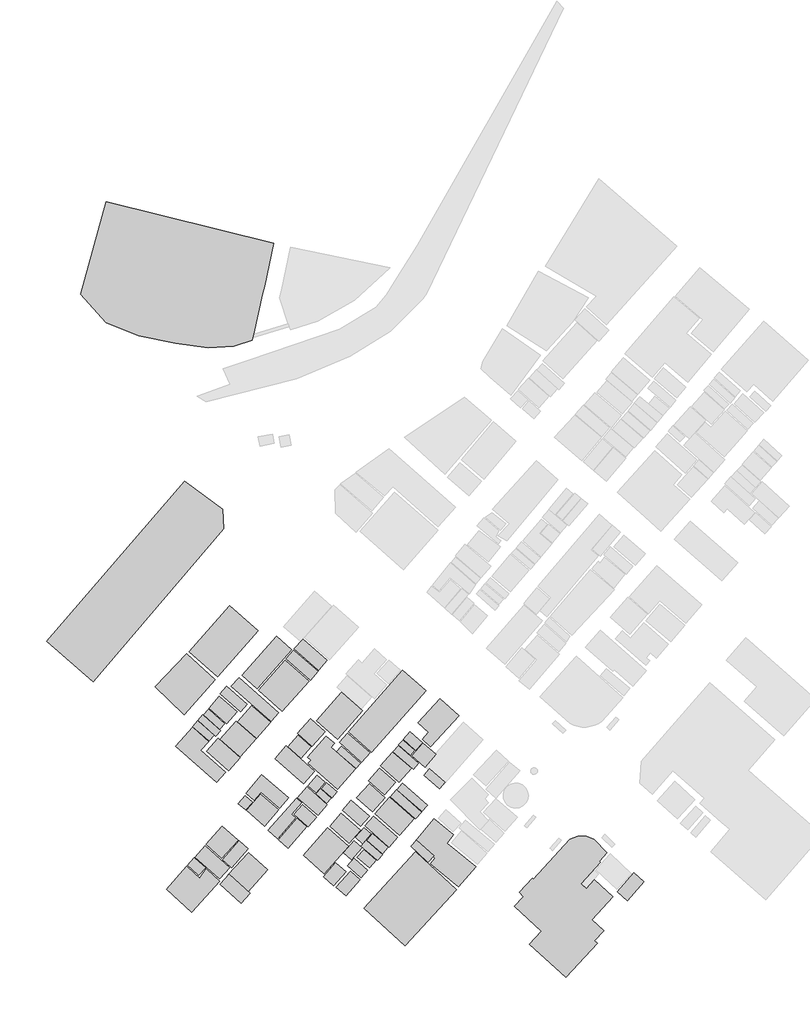
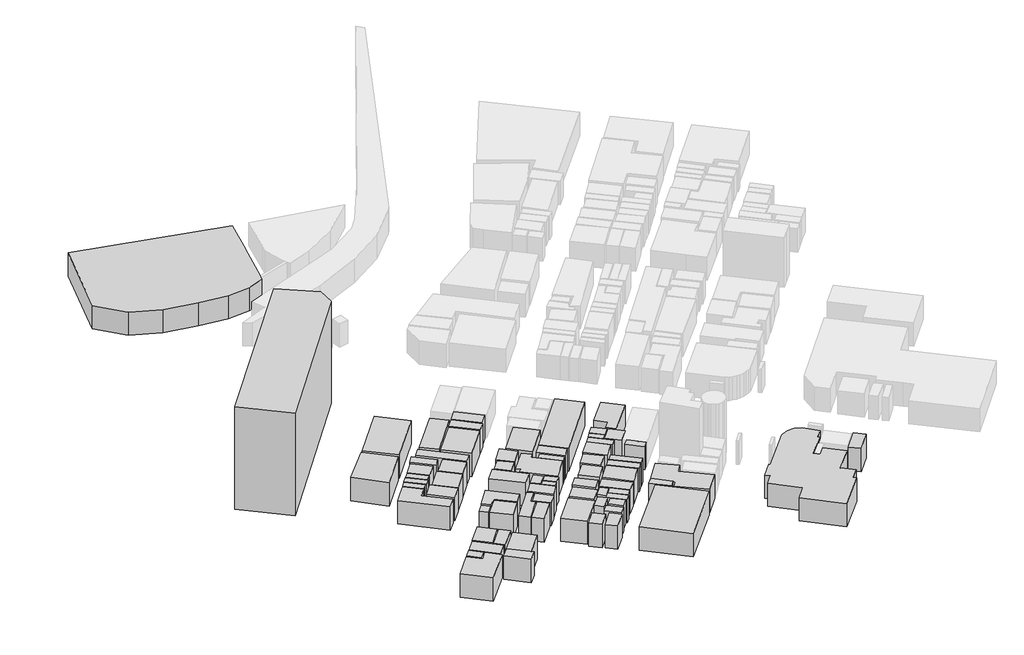
# Not in any storey, part 1 of 3: 72 proxies.
"""IFC4 building model written with IfcOpenShell, lengths in millimetres."""

from ifc_helpers import new_model, si_unit, origin, origin_with_axes, place, context, project, spatial, polyline, outline, extrude, element, save

model = new_model("IFC4")

# Units and contexts
model_context = context("Model", 3, world=origin())
ifc_project = project(units=[si_unit("LENGTHUNIT", "METRE", prefix="MILLI")], contexts=[model_context])

# Site, building
site = spatial("IfcSite", under=ifc_project)
building = spatial("IfcBuilding", under=site)

# Proxies
placement = place(None, origin())
element("IfcBuildingElementProxy", 1, Name="Mass", at=placement, inside=building, context=model_context, shape_type="SweptSolid", body=[
    extrude(outline(polyline([(-81027.0217269, 125127.6509537), (-8762.1194073, 208768.4747751), (11065.563168, 193957.3105467), (11679.8148372, 183871.9306999), (-56475.0211631, 103911.6589493), (-81027.0217269, 125127.6509537)])), origin_with_axes(), (0.0, 0.0, 1.0), 66000.0),
])
element("IfcBuildingElementProxy", 2, Name="Mass", at=placement, inside=building, context=model_context, shape_type="SweptSolid", body=[
    extrude(outline(polyline([(60169.5642931, 83373.9559982), (73321.7765149, 98307.4346465), (84306.0416675, 88633.4760284), (71144.7963334, 73699.9973801), (60169.5642931, 83373.9559982)])), origin_with_axes(), (0.0, 0.0, 1.0), 15000.0),
])
element("IfcBuildingElementProxy", 3, Name="Mass", at=placement, inside=building, context=model_context, shape_type="SweptSolid", body=[
    extrude(outline(polyline([(2438.9404523, 18836.4205741), (10893.9340249, 28276.8698459), (19105.0335488, 20926.8851949), (10650.0399787, 11475.3164303), (2438.9404523, 18836.4205741)])), origin_with_axes(), (0.0, 0.0, 1.0), 15000.0),
])
element("IfcBuildingElementProxy", 4, Name="Mass", at=placement, inside=building, context=model_context, shape_type="SweptSolid", body=[
    extrude(outline(polyline([(85191.2867223, 27565.2223158), (88867.7636278, 24318.3304577), (84405.4059075, 19258.9612947), (80728.929002, 22494.7336608), (85191.2867223, 27565.2223158)])), origin_with_axes(), (0.0, 0.0, 1.0), 15000.0),
])
element("IfcBuildingElementProxy", 5, Name="Mass", at=placement, inside=building, context=model_context, shape_type="SweptSolid", body=[
    extrude(outline(polyline([(76944.0547443, 77691.8952467), (105371.2606935, 109960.6629591), (117538.8636232, 99230.3525382), (89120.6907837, 66972.7043185), (76944.0547443, 77691.8952467)])), origin_with_axes(), (0.0, 0.0, 1.0), 15000.0),
])
element("IfcBuildingElementProxy", 6, Name="Mass", at=placement, inside=building, context=model_context, shape_type="SweptSolid", body=[
    extrude(outline(polyline([(105479.6580482, 73344.1736146), (111622.1747453, 67928.9806877), (109400.0289974, 65415.9753454), (103248.4791881, 70820.0487803), (105479.6580482, 73344.1736146)])), origin_with_axes(), (0.0, 0.0, 1.0), 15000.0),
])
element("IfcBuildingElementProxy", 7, Name="Mass", at=placement, inside=building, context=model_context, shape_type="SweptSolid", body=[
    extrude(outline(polyline([(65986.8889311, 27531.8638374), (76907.9222927, 17913.5026824), (64279.6306124, 3580.4766379), (53358.5972507, 13198.8377929), (65986.8889311, 27531.8638374)])), origin_with_axes(), (0.0, 0.0, 1.0), 15000.0),
])
element("IfcBuildingElementProxy", 8, Name="Mass", at=placement, inside=building, context=model_context, shape_type="SweptSolid", body=[
    extrude(outline(polyline([(81496.7435898, 12142.4859901), (85010.6244644, 16134.3838566), (91424.1345471, 10485.6815827), (87910.2536699, 6493.7837161), (81496.7435898, 12142.4859901)])), origin_with_axes(), (0.0, 0.0, 1.0), 15000.0),
])
element("IfcBuildingElementProxy", 9, Name="Mass", at=placement, inside=building, context=model_context, shape_type="SweptSolid", body=[
    extrude(outline(polyline([(-1878.8874617, 83362.8365054), (6657.4041263, 75834.9399721), (4082.96698, 72910.5134012), (-4453.3246055, 80427.2904425), (-1878.8874617, 83362.8365054)])), origin_with_axes(), (0.0, 0.0, 1.0), 15000.0),
])
element("IfcBuildingElementProxy", 10, Name="Mass", at=placement, inside=building, context=model_context, shape_type="SweptSolid", body=[
    extrude(outline(polyline([(3676.4769055, 89478.5574712), (12266.9671671, 81906.1829667), (9674.4637962, 78970.636903), (1083.9735346, 86543.0114075), (3676.4769055, 89478.5574712)])), origin_with_axes(), (0.0, 0.0, 1.0), 15000.0),
])
element("IfcBuildingElementProxy", 11, Name="Mass", at=placement, inside=building, context=model_context, shape_type="SweptSolid", body=[
    extrude(outline(polyline([(13179.3115586, 101509.8485342), (23883.550216, 92080.5187543), (20514.1991451, 88266.5327709), (9818.9936026, 97695.8625499), (13179.3115586, 101509.8485342)])), origin_with_axes(), (0.0, 0.0, 1.0), 15000.0),
])
element("IfcBuildingElementProxy", 12, Name="Mass", at=placement, inside=building, context=model_context, shape_type="SweptSolid", body=[
    extrude(outline(polyline([(62762.0676639, 48025.088818), (65499.1008385, 51127.4272713), (70982.2003026, 46290.4479627), (68245.167128, 43188.1095094), (62762.0676639, 48025.088818)])), origin_with_axes(), (0.0, 0.0, 1.0), 15000.0),
])
element("IfcBuildingElementProxy", 13, Name="Mass", at=placement, inside=building, context=model_context, shape_type="SweptSolid", body=[
    extrude(outline(polyline([(18174.6229327, 83262.7610719), (28625.9344316, 74066.9406383), (20342.570002, 64670.9693369), (9900.291618, 73877.9092632), (18174.6229327, 83262.7610719)])), origin_with_axes(), (0.0, 0.0, 1.0), 15000.0),
])
element("IfcBuildingElementProxy", 14, Name="Mass", at=placement, inside=building, context=model_context, shape_type="SweptSolid", body=[
    extrude(outline(polyline([(109689.0886075, 17835.6662344), (112670.0158283, 21093.6775845), (121685.0623915, 12843.0140274), (118695.1020584, 9585.0026774), (109689.0886075, 17835.6662344)])), origin_with_axes(), (0.0, 0.0, 1.0), 15000.0),
])
element("IfcBuildingElementProxy", 15, Name="Mass", at=placement, inside=building, context=model_context, shape_type="SweptSolid", body=[
    extrude(outline(polyline([(76537.5646672, 7572.3745045), (79961.1144168, 11464.1969375), (87043.0748422, 5226.1615525), (83619.5250952, 1334.3391203), (76537.5646672, 7572.3745045)])), origin_with_axes(), (0.0, 0.0, 1.0), 15000.0),
])
element("IfcBuildingElementProxy", 16, Name="Mass", at=placement, inside=building, context=model_context, shape_type="SweptSolid", body=[
    extrude(outline(polyline([(23630.6230575, 36694.3257933), (31064.8748838, 45134.0207255), (40432.212848, 36883.3571684), (32997.9610217, 28443.6622362), (23630.6230575, 36694.3257933)])), origin_with_axes(), (0.0, 0.0, 1.0), 15000.0),
])
element("IfcBuildingElementProxy", 17, Name="Mass", at=placement, inside=building, context=model_context, shape_type="SweptSolid", body=[
    extrude(outline(polyline([(78271.9223252, 41931.6068378), (87919.2867847, 33436.3144425), (83393.697276, 28299.1088315), (73737.2997043, 36794.4012269), (78271.9223252, 41931.6068378)])), origin_with_axes(), (0.0, 0.0, 1.0), 15000.0),
])
element("IfcBuildingElementProxy", 18, Name="Mass", at=placement, inside=building, context=model_context, shape_type="SweptSolid", body=[
    extrude(outline(polyline([(93673.3796317, 59833.9900274), (100095.9228241, 67128.3772152), (109851.6846383, 58533.0093863), (103429.1414434, 51238.6221977), (93673.3796317, 59833.9900274)])), origin_with_axes(), (0.0, 0.0, 1.0), 15000.0),
])
element("IfcBuildingElementProxy", 19, Name="Mass", at=placement, inside=building, context=model_context, shape_type="SweptSolid", body=[
    extrude(outline(polyline([(116572.320553, 55063.7276747), (119408.7179701, 58288.3805472), (127366.890338, 51271.9806761), (124521.4598087, 48047.3278036), (116572.320553, 55063.7276747)])), origin_with_axes(), (0.0, 0.0, 1.0), 15000.0),
])
element("IfcBuildingElementProxy", 20, Name="Mass", at=placement, inside=building, context=model_context, shape_type="SweptSolid", body=[
    extrude(outline(polyline([(85516.4787814, 28499.2596994), (90069.1676269, 33658.7042952), (102688.4261949, 22539.2116311), (98135.7373495, 17379.7670346), (85516.4787814, 28499.2596994)])), origin_with_axes(), (0.0, 0.0, 1.0), 15000.0),
])
element("IfcBuildingElementProxy", 21, Name="Mass", at=placement, inside=building, context=model_context, shape_type="SweptSolid", body=[
    extrude(outline(polyline([(40350.9148326, 21360.5454084), (50052.4779682, 32379.9626388), (55065.8555668, 27954.4045588), (45364.2924312, 16934.9873283), (40350.9148326, 21360.5454084)])), origin_with_axes(), (0.0, 0.0, 1.0), 15000.0),
])
element("IfcBuildingElementProxy", 22, Name="Mass", at=placement, inside=building, context=model_context, shape_type="SweptSolid", body=[
    extrude(outline(polyline([(45490.7560105, 69930.489367), (50720.928316, 75868.2984497), (57504.7960191, 69897.1308886), (52265.5906013, 63959.321806), (45490.7560105, 69930.489367)])), origin_with_axes(), (0.0, 0.0, 1.0), 15000.0),
])
element("IfcBuildingElementProxy", 23, Name="Mass", at=placement, inside=building, context=model_context, shape_type="SweptSolid", body=[
    extrude(outline(polyline([(29818.3053184, 99430.5034061), (43693.1665642, 115175.7050189), (56222.0940046, 104134.0488028), (42347.2327588, 88388.84719), (29818.3053184, 99430.5034061)])), origin_with_axes(), (0.0, 0.0, 1.0), 15000.0),
])
element("IfcBuildingElementProxy", 24, Name="Mass", at=placement, inside=building, context=model_context, shape_type="SweptSolid", body=[
    extrude(outline(polyline([(55743.3390269, 49526.2203279), (60585.0874824, 55019.2497043), (64785.4849294, 51316.4586465), (59943.7364739, 45823.4292708), (55743.3390269, 49526.2203279)])), origin_with_axes(), (0.0, 0.0, 1.0), 15000.0),
])
element("IfcBuildingElementProxy", 25, Name="Mass", at=placement, inside=building, context=model_context, shape_type="SweptSolid", body=[
    extrude(outline(polyline([(76546.5977821, 77024.7256869), (88226.4126193, 66728.0754794), (83926.6509298, 61846.6182003), (72237.8029803, 72143.268407), (76546.5977821, 77024.7256869)])), origin_with_axes(), (0.0, 0.0, 1.0), 15000.0),
])
element("IfcBuildingElementProxy", 26, Name="Mass", at=placement, inside=building, context=model_context, shape_type="SweptSolid", body=[
    extrude(outline(polyline([(19637.9872051, 105991.0040781), (40396.0803965, 87699.4386447), (36439.5769931, 83207.1636087), (15681.4838018, 101498.7290414), (19637.9872051, 105991.0040781)])), origin_with_axes(), (0.0, 0.0, 1.0), 15000.0),
])
element("IfcBuildingElementProxy", 27, Name="Mass", at=placement, inside=building, context=model_context, shape_type="SweptSolid", body=[
    extrude(outline(polyline([(44334.5175727, 115909.5915346), (48318.1203128, 120424.1055562), (60991.5775569, 109260.134921), (57007.9748169, 104734.5014066), (44334.5175727, 115909.5915346)])), origin_with_axes(), (0.0, 0.0, 1.0), 15000.0),
])
element("IfcBuildingElementProxy", 28, Name="Mass", at=placement, inside=building, context=model_context, shape_type="SweptSolid", body=[
    extrude(outline(polyline([(98903.5519373, 43821.9205908), (101974.8102858, 47302.3217951), (115099.9231684, 35738.049424), (112028.6648198, 32257.6482197), (98903.5519373, 43821.9205908)])), origin_with_axes(), (0.0, 0.0, 1.0), 15000.0),
])
element("IfcBuildingElementProxy", 29, Name="Mass", at=placement, inside=building, context=model_context, shape_type="SweptSolid", body=[
    extrude(outline(polyline([(226171.0780354, 3936.3004034), (231446.4159048, -611.5720966), (222837.8594161, -10607.9960018), (217562.5215467, -6060.1235018), (226171.0780354, 3936.3004034)])), origin_with_axes(), (0.0, 0.0, 1.0), 15000.0),
])
element("IfcBuildingElementProxy", 30, Name="Mass", at=placement, inside=building, context=model_context, shape_type="SweptSolid", body=[
    extrude(outline(polyline([(14118.7552895, 2902.1875854), (24624.2654644, 14566.5353908), (34614.8882101, 5570.8658252), (24100.3449229, -6093.4819802), (14118.7552895, 2902.1875854)])), origin_with_axes(), (0.0, 0.0, 1.0), 15000.0),
])
element("IfcBuildingElementProxy", 31, Name="Mass", at=placement, inside=building, context=model_context, shape_type="SweptSolid", body=[
    extrude(outline(polyline([(67829.6439386, 69685.8605287), (80647.6309891, 58388.4559815), (71171.8956702, 47635.906575), (55842.7032668, 61134.9706694), (57324.1337637, 62814.0140616), (55499.4449806, 64426.3404978), (65246.17368, 75490.2356994), (69573.0347063, 71676.2497152), (67829.6439386, 69685.8605287)])), origin_with_axes(), (0.0, 0.0, 1.0), 15000.0),
])
element("IfcBuildingElementProxy", 32, Name="Mass", at=placement, inside=building, context=model_context, shape_type="SweptSolid", body=[
    extrude(outline(polyline([(19773.4838966, 20660.017371), (24488.7687729, 16434.6101581), (15726.6493656, 6649.4566136), (11011.3644894, 10874.8638257), (19773.4838966, 20660.017371)])), origin_with_axes(), (0.0, 0.0, 1.0), 15000.0),
])
element("IfcBuildingElementProxy", 33, Name="Mass", at=placement, inside=building, context=model_context, shape_type="SweptSolid", body=[
    extrude(outline(polyline([(9773.8280387, -1968.1502017), (14498.1460273, 3269.1308436), (25554.676083, -6682.8150912), (20830.3580919, -11931.2156285), (9773.8280387, -1968.1502017)])), origin_with_axes(), (0.0, 0.0, 1.0), 15000.0),
])
element("IfcBuildingElementProxy", 34, Name="Mass", at=placement, inside=building, context=model_context, shape_type="SweptSolid", body=[
    extrude(outline(polyline([(-3251.9206065, 12164.7249749), (2005.3510384, 18035.8171024), (14769.1394103, 6616.0981352), (9502.8346531, 733.8865157), (-3251.9206065, 12164.7249749)])), origin_with_axes(), (0.0, 0.0, 1.0), 15000.0),
])
element("IfcBuildingElementProxy", 35, Name="Mass", at=placement, inside=building, context=model_context, shape_type="SweptSolid", body=[
    extrude(outline(polyline([(74478.0149527, 14410.8624933), (79961.1144168, 20626.6588926), (83989.8827207, 17079.5407331), (78506.7832566, 10863.7443337), (74478.0149527, 14410.8624933)])), origin_with_axes(), (0.0, 0.0, 1.0), 15000.0),
])
element("IfcBuildingElementProxy", 36, Name="Mass", at=placement, inside=building, context=model_context, shape_type="SweptSolid", body=[
    extrude(outline(polyline([(8689.8545041, 74267.0915063), (20152.8746344, 64092.7557179), (14227.1526442, 57421.0601195), (2773.1656262, 67595.3959079), (8689.8545041, 74267.0915063)])), origin_with_axes(), (0.0, 0.0, 1.0), 15000.0),
])
element("IfcBuildingElementProxy", 37, Name="Mass", at=placement, inside=building, context=model_context, shape_type="SweptSolid", body=[
    extrude(outline(polyline([(110140.7442484, 65137.9880287), (116048.4000115, 71843.0421055), (122832.2677171, 65871.8745445), (116915.5788392, 59155.7009749), (110140.7442484, 65137.9880287)])), origin_with_axes(), (0.0, 0.0, 1.0), 15000.0),
])
element("IfcBuildingElementProxy", 38, Name="Mass", at=placement, inside=building, context=model_context, shape_type="SweptSolid", body=[
    extrude(outline(polyline([(73186.2798234, 34993.0434155), (83213.0350207, 26164.1662395), (77251.1805789, 19392.3952067), (67224.4253817, 28232.3918755), (73186.2798234, 34993.0434155)])), origin_with_axes(), (0.0, 0.0, 1.0), 15000.0),
])
element("IfcBuildingElementProxy", 39, Name="Mass", at=placement, inside=building, context=model_context, shape_type="SweptSolid", body=[
    extrude(outline(polyline([(109165.168066, 77736.3732178), (115614.8105976, 72054.3124663), (112118.9959475, 68084.6535845), (105678.3865281, 73766.7143361), (109165.168066, 77736.3732178)])), origin_with_axes(), (0.0, 0.0, 1.0), 15000.0),
])
element("IfcBuildingElementProxy", 40, Name="Mass", at=placement, inside=building, context=model_context, shape_type="SweptSolid", body=[
    extrude(outline(polyline([(70530.5446642, -3591.5961307), (77946.7302635, 4825.8598167), (83131.7370052, 255.7483319), (75715.5514034, -8150.5881227), (70530.5446642, -3591.5961307)])), origin_with_axes(), (0.0, 0.0, 1.0), 15000.0),
])
element("IfcBuildingElementProxy", 41, Name="Mass", at=placement, inside=building, context=model_context, shape_type="SweptSolid", body=[
    extrude(outline(polyline([(59988.9020377, 45211.8571742), (62328.4782501, 47880.5354133), (67947.0744056, 42932.3611775), (65598.465081, 40263.6829384), (59988.9020377, 45211.8571742)])), origin_with_axes(), (0.0, 0.0, 1.0), 15000.0),
])
element("IfcBuildingElementProxy", 42, Name="Mass", at=placement, inside=building, context=model_context, shape_type="SweptSolid", body=[
    extrude(outline(polyline([(776.8477, 86565.2503931), (10071.9207611, 78381.303792), (7506.516727, 75467.9967139), (-1788.5563341, 83651.9433149), (776.8477, 86565.2503931)])), origin_with_axes(), (0.0, 0.0, 1.0), 15000.0),
])
element("IfcBuildingElementProxy", 43, Name="Mass", at=placement, inside=building, context=model_context, shape_type="SweptSolid", body=[
    extrude(outline(polyline([(89662.6775523, 24329.4499497), (97629.8830325, 17313.0500786), (94694.1213755, 13988.3217718), (86735.9490076, 21004.7216437), (89662.6775523, 24329.4499497)])), origin_with_axes(), (0.0, 0.0, 1.0), 15000.0),
])
element("IfcBuildingElementProxy", 44, Name="Mass", at=placement, inside=building, context=model_context, shape_type="SweptSolid", body=[
    extrude(outline(polyline([(48471.6832288, 34648.3391428), (52897.9084975, 39674.3498266), (60377.3258878, 33080.490677), (55951.100619, 28054.4799924), (48471.6832288, 34648.3391428)])), origin_with_axes(), (0.0, 0.0, 1.0), 15000.0),
])
element("IfcBuildingElementProxy", 45, Name="Mass", at=placement, inside=building, context=model_context, shape_type="SweptSolid", body=[
    extrude(outline(polyline([(83664.690659, 17957.9806536), (86257.1940299, 20904.6462093), (94838.6511818, 13343.3911976), (92246.1478109, 10407.8451339), (83664.690659, 17957.9806536)])), origin_with_axes(), (0.0, 0.0, 1.0), 15000.0),
])
element("IfcBuildingElementProxy", 46, Name="Mass", at=placement, inside=building, context=model_context, shape_type="SweptSolid", body=[
    extrude(outline(polyline([(118966.095444, 77458.3859011), (113392.6648523, 82495.5160777), (124801.4863065, 95105.0207596), (134665.6454729, 86176.06815), (119932.6385116, 69908.2503814), (115650.9430492, 73788.9533216), (118966.095444, 77458.3859011)])), origin_with_axes(), (0.0, 0.0, 1.0), 15000.0),
])
element("IfcBuildingElementProxy", 47, Name="Mass", at=placement, inside=building, context=model_context, shape_type="SweptSolid", body=[
    extrude(outline(polyline([(38508.1598225, 63647.9760117), (44379.6831365, 70308.5521173), (59320.4516899, 57131.95331), (53457.9614906, 50471.3772044), (38508.1598225, 63647.9760117)])), origin_with_axes(), (0.0, 0.0, 1.0), 15000.0),
])
element("IfcBuildingElementProxy", 48, Name="Mass", at=placement, inside=building, context=model_context, shape_type="SweptSolid", body=[
    extrude(outline(polyline([(49781.4845852, 42943.4806703), (52482.3853082, 40552.7897479), (47198.0143266, 34559.3832013), (49347.8951713, 32669.0694483), (39845.0605156, 21883.1615642), (34994.2789478, 26153.0467467), (49781.4845852, 42943.4806703)])), origin_with_axes(), (0.0, 0.0, 1.0), 15000.0),
])
element("IfcBuildingElementProxy", 49, Name="Mass", at=placement, inside=building, context=model_context, shape_type="SweptSolid", body=[
    extrude(outline(polyline([(122208.9829356, 11642.1088198), (111811.8701129, 20170.7596936), (121730.2279579, 32257.6482197), (132027.9765382, 23873.5507507), (128432.7976481, 19447.9926706), (143716.8244877, 7094.2363199), (134575.3143452, -3269.1308428), (119878.4398355, 8806.6381905), (122208.9829356, 11642.1088198)])), origin_with_axes(), (0.0, 0.0, 1.0), 15000.0),
])
element("IfcBuildingElementProxy", 50, Name="Mass", at=placement, inside=building, context=model_context, shape_type="SweptSolid", body=[
    extrude(outline(polyline([(23359.6296744, 45678.8758661), (31498.4642977, 55341.7149914), (45617.2195872, 43165.8705238), (40847.7360348, 37750.6775961), (31272.6364785, 46190.3725283), (27614.2257975, 42031.6822722), (23359.6296744, 45678.8758661)])), origin_with_axes(), (0.0, 0.0, 1.0), 15000.0),
])
element("IfcBuildingElementProxy", 51, Name="Mass", at=placement, inside=building, context=model_context, shape_type="SweptSolid", body=[
    extrude(outline(polyline([(103185.2473997, 70519.822478), (113699.7906869, 61257.2850885), (110890.4926091, 58065.9906937), (100366.9162097, 67328.5280832), (103185.2473997, 70519.822478)])), origin_with_axes(), (0.0, 0.0, 1.0), 15000.0),
])
element("IfcBuildingElementProxy", 52, Name="Mass", at=placement, inside=building, context=model_context, shape_type="SweptSolid", body=[
    extrude(outline(polyline([(90873.1146662, 34726.1755916), (98506.094975, 43388.2603773), (111224.717783, 32190.9312637), (103591.7374742, 23517.7269852), (90873.1146662, 34726.1755916)])), origin_with_axes(), (0.0, 0.0, 1.0), 15000.0),
])
element("IfcBuildingElementProxy", 53, Name="Mass", at=placement, inside=building, context=model_context, shape_type="SweptSolid", body=[
    extrude(outline(polyline([(87530.8629347, 52072.5841478), (93339.1544578, 58655.3238055), (101631.5519996, 51349.8171249), (95823.2604739, 44767.0774672), (87530.8629347, 52072.5841478)])), origin_with_axes(), (0.0, 0.0, 1.0), 15000.0),
])
element("IfcBuildingElementProxy", 54, Name="Mass", at=placement, inside=building, context=model_context, shape_type="SweptSolid", body=[
    extrude(outline(polyline([(102453.5652635, 47457.9946919), (105308.0289051, 50704.8865499), (118252.4795323, 39307.4065692), (115388.9827785, 36060.5147111), (102453.5652635, 47457.9946919)])), origin_with_axes(), (0.0, 0.0, 1.0), 15000.0),
])
element("IfcBuildingElementProxy", 55, Name="Mass", at=placement, inside=building, context=model_context, shape_type="SweptSolid", body=[
    extrude(outline(polyline([(63873.1405379, 1957.0307089), (70268.5843935, 9218.0594191), (75625.2202757, 4503.3945296), (69229.7764227, -2757.6341806), (63873.1405379, 1957.0307089)])), origin_with_axes(), (0.0, 0.0, 1.0), 15000.0),
])
element("IfcBuildingElementProxy", 56, Name="Mass", at=placement, inside=building, context=model_context, shape_type="SweptSolid", body=[
    extrude(outline(polyline([(-6521.9074348, 119601.2630989), (14687.8413948, 143719.4426887), (29718.9410784, 130498.3659102), (8518.225361, 106380.1863212), (-6521.9074348, 119601.2630989)])), origin_with_axes(), (0.0, 0.0, 1.0), 15000.0),
])
element("IfcBuildingElementProxy", 57, Name="Mass", at=placement, inside=building, context=model_context, shape_type="SweptSolid", body=[
    extrude(outline(polyline([(-7596.8478572, 118411.4773841), (7090.9935402, 105034.7277089), (-9069.2452419, 86698.684305), (-24145.5104893, 101220.7417247), (-7596.8478572, 118411.4773841)])), origin_with_axes(), (0.0, 0.0, 1.0), 15000.0),
])
element("IfcBuildingElementProxy", 58, Name="Mass", at=placement, inside=building, context=model_context, shape_type="SweptSolid", body=[
    extrude(outline(polyline([(81270.9157706, 43132.5120454), (87865.088106, 50615.9306091), (96211.6843239, 43254.8264653), (89617.5119885, 35771.4079016), (81270.9157706, 43132.5120454)])), origin_with_axes(), (0.0, 0.0, 1.0), 15000.0),
])
element("IfcBuildingElementProxy", 59, Name="Mass", at=placement, inside=building, context=model_context, shape_type="SweptSolid", body=[
    extrude(outline(polyline([(9349.2717371, 96250.328504), (18581.1130073, 88110.8598733), (13179.3115586, 81984.0194155), (3947.4702885, 90123.4880454), (9349.2717371, 96250.328504)])), origin_with_axes(), (0.0, 0.0, 1.0), 15000.0),
])
element("IfcBuildingElementProxy", 60, Name="Mass", at=placement, inside=building, context=model_context, shape_type="SweptSolid", body=[
    extrude(outline(polyline([(26295.3913315, 91346.6322386), (36087.2855947, 82717.9059313), (28806.5966869, 74445.0033886), (19005.6693089, 83084.8491887), (26295.3913315, 91346.6322386)])), origin_with_axes(), (0.0, 0.0, 1.0), 15000.0),
])
element("IfcBuildingElementProxy", 61, Name="Mass", at=placement, inside=building, context=model_context, shape_type="SweptSolid", body=[
    extrude(outline(polyline([(50422.8355937, 43321.5434213), (55327.8158376, 48881.2897529), (65860.4253518, 39607.6328707), (60955.4451054, 34036.7670462), (50422.8355937, 43321.5434213)])), origin_with_axes(), (0.0, 0.0, 1.0), 15000.0),
])
element("IfcBuildingElementProxy", 62, Name="Mass", at=placement, inside=building, context=model_context, shape_type="SweptSolid", body=[
    extrude(outline(polyline([(73267.5778389, 70075.0427718), (83249.1674722, 61279.5240741), (80837.3263567, 58533.0093863), (70846.7036111, 67328.5280832), (73267.5778389, 70075.0427718)])), origin_with_axes(), (0.0, 0.0, 1.0), 15000.0),
])
element("IfcBuildingElementProxy", 63, Name="Mass", at=placement, inside=building, context=model_context, shape_type="SweptSolid", body=[
    extrude(outline(polyline([(50323.4713512, 76980.2477165), (57044.1072684, 84619.339177), (64749.3524778, 77836.4486514), (58019.6834483, 70197.3571909), (50323.4713512, 76980.2477165)])), origin_with_axes(), (0.0, 0.0, 1.0), 15000.0),
])
element("IfcBuildingElementProxy", 64, Name="Mass", at=placement, inside=building, context=model_context, shape_type="SweptSolid", body=[
    extrude(outline(polyline([(21318.1461844, 107180.7897929), (39275.9744102, 127573.9393392), (47225.1136659, 120568.6589609), (29267.2854375, 100175.5094146), (21318.1461844, 107180.7897929)])), origin_with_axes(), (0.0, 0.0, 1.0), 15000.0),
])
element("IfcBuildingElementProxy", 65, Name="Mass", at=placement, inside=building, context=model_context, shape_type="SweptSolid", body=[
    extrude(outline(polyline([(48625.2461474, 121024.55816), (53196.0012199, 126217.3612341), (65842.3591247, 115075.6295845), (61271.6040522, 109893.9460032), (48625.2461474, 121024.55816)])), origin_with_axes(), (0.0, 0.0, 1.0), 15000.0),
])
element("IfcBuildingElementProxy", 66, Name="Mass", at=placement, inside=building, context=model_context, shape_type="SweptSolid", body=[
    extrude(outline(polyline([(205476.2166324, 21605.1742475), (212242.0181135, 14544.2964052), (208186.1504702, 10118.7383252), (208890.7332671, 9473.8077502), (198574.9184624, -1767.9993338), (201330.0178615, -4292.1241681), (205521.3821962, 266.8678239), (215259.0777834, -8662.0847857), (204329.0113094, -20582.1809215), (210588.9584709, -26319.8391362), (205738.1769032, -31612.7176447), (207111.2100479, -32869.2203163), (190716.1103344, -50749.3645203), (171719.4741378, -33336.2390081), (177979.4212993, -26497.7510193), (163905.8315736, -13588.0200359), (168612.0833377, -8450.814425), (166299.6064621, -6326.9913257), (173119.6066193, 1111.9492668), (173679.6596124, 600.4526038), (192847.9249521, 21405.0233796), (196930.8919321, 23039.5888014), (201339.0509737, 23117.4252493), (205476.2166324, 21605.1742475)])), origin_with_axes(), (0.0, 0.0, 1.0), 15000.0),
])
element("IfcBuildingElementProxy", 67, Name="Mass", at=placement, inside=building, context=model_context, shape_type="SweptSolid", body=[
    extrude(outline(polyline([(-18264.954063, -4692.4259039), (-7831.7087886, 7472.2990709), (-894.278167, 1145.3077444), (2574.4371438, 6015.6455315), (9611.2320079, -333.5847799), (-5040.4769379, -16601.4025477), (-18264.954063, -4692.4259039)])), origin_with_axes(), (0.0, 0.0, 1.0), 15000.0),
])
element("IfcBuildingElementProxy", 68, Name="Mass", at=placement, inside=building, context=model_context, shape_type="SweptSolid", body=[
    extrude(outline(polyline([(7931.0730286, 51238.6221977), (-13378.0400436, 70163.9987133), (-8716.9538434, 75412.3992507), (-4670.1193124, 79960.2717506), (3757.7749209, 72476.8531869), (-289.0596101, 67928.9806877), (12592.1592288, 56475.903243), (7931.0730286, 51238.6221977)])), origin_with_axes(), (0.0, 0.0, 1.0), 15000.0),
])
element("IfcBuildingElementProxy", 69, Name="Mass", at=placement, inside=building, context=model_context, shape_type="SweptSolid", body=[
    extrude(outline(polyline([(85064.8231431, -14466.4599564), (112010.5985953, 14977.9566194), (133563.6057112, -4759.1428599), (106617.8302589, -34203.5594358), (85064.8231431, -14466.4599564)])), origin_with_axes(), (0.0, 0.0, 1.0), 15000.0),
])
element("IfcBuildingElementProxy", 70, Name="Mass", at=placement, inside=building, context=model_context, shape_type="SweptSolid", body=[
    extrude(outline(polyline([(19195.364679, 40196.9659824), (22871.8415845, 44377.8952242), (26719.9476331, 40986.4499614), (23043.470725, 36816.6402124), (19195.364679, 40196.9659824)])), origin_with_axes(), (0.0, 0.0, 1.0), 15000.0),
])
element("IfcBuildingElementProxy", 71, Name="Mass", at=placement, inside=building, context=model_context, shape_type="SweptSolid", body=[
    extrude(outline(polyline([(-63087.2597256, 306408.7398618), (-49898.9150522, 354911.9668645), (37704.2127857, 333195.5976906), (32952.7954578, 310778.7004794), (31968.1861631, 306931.3560176), (27442.5966544, 285726.483506), (26927.7092252, 283791.6917827), (26503.1529236, 282535.1891111), (16801.589788, 279299.4167459), (3595.1788901, 278498.8132742), (-13459.338059, 280822.7872413), (-32844.3981056, 284703.4901807), (-49898.9150522, 291675.4120815), (-63087.2597256, 306408.7398618)])), origin_with_axes(), (0.0, 0.0, 1.0), 15000.0),
])
element("IfcBuildingElementProxy", 72, Name="Mass", at=placement, inside=building, context=model_context, shape_type="SweptSolid", body=[
    extrude(outline(polyline([(-1436.2649356, 2746.5146886), (-7235.5233465, 8028.2737043), (-3730.6755841, 11931.2156293), (2104.7152783, 6693.934584), (-1436.2649356, 2746.5146886)])), origin_with_axes(), (0.0, 0.0, 1.0), 15000.0),
])

save(model, "model.ifc")

# Revit data of these elements
# Project information
#   プロジェクト発行日 = "発行日"
#   プロジェクト ステータス = "プロジェクト ステータス"
#   クライアント名 = "オーナ"
#   計画地住所 = "ここにアドレスを入力"
#   プロジェクト名 = "プロジェクト名"
#   プロジェクト番号 = "0001"
# Elements 1, 2, 3, 4, 5, 6, 7, 8, 9, 10, 11, 12, 13, 14, 15, 16, 17, 18, 19, 20, 21, 22, 23, 24, 25, 26, 27, 28, 29, 30, 31, 32, 33, 34, 35, 36, 37, 38, 39, 40, 41, 42, 43, 44, 45, 46, 47, 48, 49, 50, 51, 52, 53, 54, 55, 56, 57, 58, 59, 60, 61, 62, 63, 64, 65, 66, 67, 68, 69, 70, 71, 72 (IfcBuildingElementProxy)
#   Phase Created = 新しい建設
#   Materials on its faces: "周辺建物"
# Materials
#   "周辺建物": class "一般", colour RGB 120 120 120, transparency 0, Cost = 0
